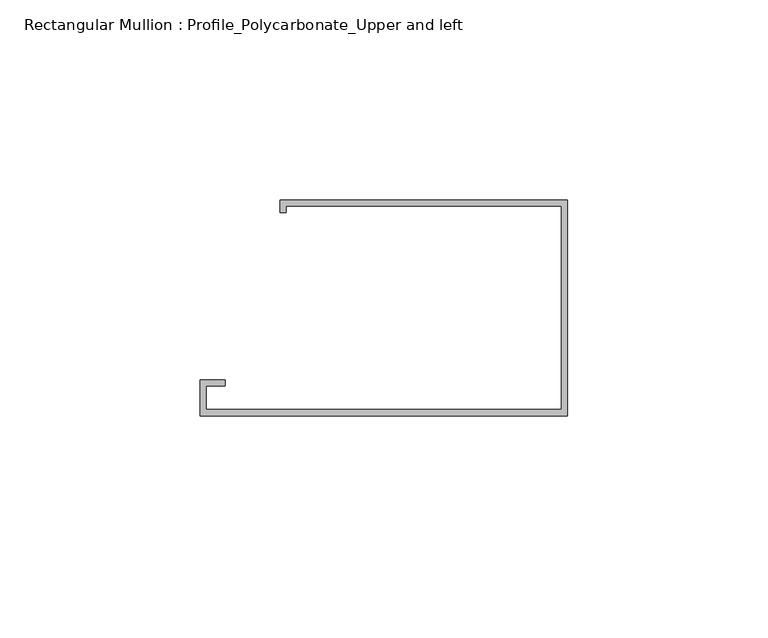
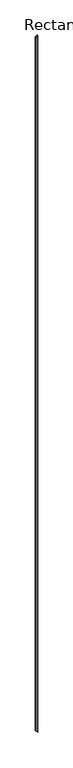
"""IFC4 building model written with IfcOpenShell, lengths in millimetres: member geometry, Rectangular Mullion : Profile_Polycarbonate_Upper and left."""

from ifc_helpers import new_model, si_unit, origin, place, context, project, spatial, faceted_brep, source, transform, mapped, element, save


def rectangular_mullion_profile_polycarbonate_upper_and_left_a248562a(model_context):
    return source(origin(), model_context, "Body", "Brep", [
        faceted_brep([(0.0, 25.015825, 0.0), (0.0, -28.984575, 0.0), (0.0, -28.984575, -31651.7402253), (0.0, 25.015825, -31651.7402253), (-71.9836, 25.015825, -69.046742), (-71.9836, 25.015825, -31576.6948499), (-71.9836, 21.840825, -69.046742), (-71.9836, 21.840825, -31576.6948499), (-70.3961, 21.840825, -67.5240104), (-70.3961, 21.840825, -31578.3498732), (-70.3961, 23.428325, -67.5240104), (-70.3961, 23.428325, -31578.3498732), (-1.5875, 23.428325, -1.5227316), (-1.5875, 23.428325, -31650.085202), (-1.5875, -27.397075, -1.5227316), (-1.5875, -27.397075, -31650.085202), (-90.4113, -27.397075, -86.7226105), (-90.4113, -27.397075, -31557.4833398), (-90.4113, -21.580475, -86.7226105), (-90.4113, -21.580475, -31557.4833398), (-85.6488, -21.580475, -82.1544157), (-85.6488, -21.580475, -31562.4484096), (-85.6488, -19.992975, -82.1544157), (-85.6488, -19.992975, -31562.4484096), (-91.9988, -19.992975, -88.2453421), (-91.9988, -19.992975, -31555.8283165), (-91.9988, -28.984575, -88.2453421), (-91.9988, -28.984575, -31555.8283165)], [[[0, 1, 2, 3]], [[4, 0, 3, 5]], [[6, 4, 5, 7]], [[8, 6, 7, 9]], [[10, 8, 9, 11]], [[12, 10, 11, 13]], [[14, 12, 13, 15]], [[16, 14, 15, 17]], [[18, 16, 17, 19]], [[20, 18, 19, 21]], [[22, 20, 21, 23]], [[24, 22, 23, 25]], [[26, 24, 25, 27]], [[1, 26, 27, 2]], [[1, 0, 4, 6, 8, 10, 12, 14, 16, 18, 20, 22, 24, 26]], [[2, 27, 25, 23, 21, 19, 17, 15, 13, 11, 9, 7, 5, 3]]]),
    ])


if __name__ == "__main__":
    model = new_model("IFC4")
    model_context = context("Model", 3, world=origin())
    ifc_project = project(units=[si_unit("LENGTHUNIT", "METRE", prefix="MILLI")], contexts=[model_context])
    site = spatial("IfcSite", under=ifc_project)
    building = spatial("IfcBuilding", under=site)
    placement = place(None, origin())
    rectangular_mullion_profile_polycarbonate_upper_and_left_shape = rectangular_mullion_profile_polycarbonate_upper_and_left_a248562a(model_context)
    element("IfcMember", 1, ObjectType="Rectangular Mullion : Profile_Polycarbonate_Upper and left", at=placement, inside=building, context=model_context, shape_type="MappedRepresentation", body=[
        mapped(rectangular_mullion_profile_polycarbonate_upper_and_left_shape, transform((0.0, 0.0, 0.0), x_axis=(1.0, 0.0, 0.0), y_axis=(0.0, 1.0, 0.0), z_axis=(0.0, 0.0, 1.0))),
    ])
    save(model, "model.ifc")

# Revit data of these elements
# Type "Rectangular Mullion : Profile_Polycarbonate_Upper and left"
#   built-in parameter 1007322 = 0.177167 (stored number, unit not read)
#   built-in parameter 1007321 = 0.00520833 (stored number, unit not read)
#   built-in parameter 1007320 = 0 (stored number, unit not read)
